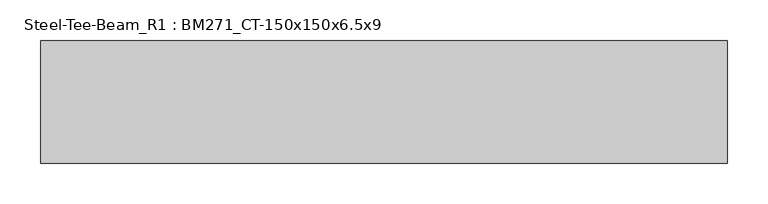
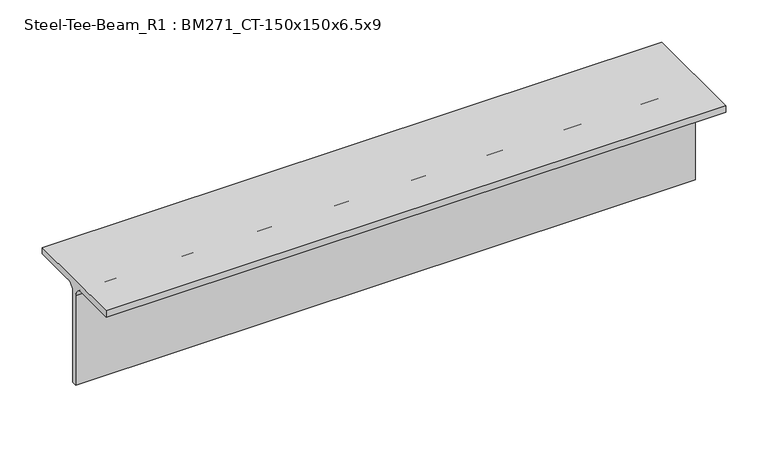
"""IFC4 building model written with IfcOpenShell, lengths in millimetres: member geometry, Steel-Tee-Beam_R1 : BM271_CT-150x150x6.5x9."""

from ifc_helpers import new_model, si_unit, point, frame, frame_2d, origin, place, context, project, spatial, polyline, circle_curve, trimmed, segment, composite_curve, outline, extrude, source, transform, mapped, element, save


def steel_tee_beam_r1_bm271_ct_150x150x6_5x9_ef0092a5(model_context):
    return source(origin(), model_context, "Body", "SweptSolid", [
        extrude(outline(composite_curve([segment(polyline([(75.0, 75.0), (75.0, 66.0), (16.25, 66.0)]), True, "CONTINUOUS"), segment(trimmed(circle_curve(frame_2d((16.25, 53.0)), 13.0), [point((16.25, 66.0))], [point((3.25, 53.0))], True, "CARTESIAN"), True, "CONTINUOUS"), segment(polyline([(3.25, 53.0), (3.25, -75.0), (-3.25, -75.0), (-3.25, 53.0)]), True, "CONTINUOUS"), segment(trimmed(circle_curve(frame_2d((-16.25, 53.0)), 13.0), [point((-3.25, 53.0))], [point((-16.25, 66.0))], True, "CARTESIAN"), True, "CONTINUOUS"), segment(polyline([(-16.25, 66.0), (-75.0, 66.0), (-75.0, 75.0), (75.0, 75.0)]), True, "CONTINUOUS")], self_intersect=False)), frame((-500.0, 0.0, 0.0), z_axis=(1.0, 0.0, 0.0), x_axis=(0.0, 1.0, 0.0)), (0.0, 0.0, 1.0), 841.5608007),
    ])


if __name__ == "__main__":
    model = new_model("IFC4")
    model_context = context("Model", 3, world=origin())
    ifc_project = project(units=[si_unit("LENGTHUNIT", "METRE", prefix="MILLI")], contexts=[model_context])
    site = spatial("IfcSite", under=ifc_project)
    building = spatial("IfcBuilding", under=site)
    placement = place(None, origin())
    steel_tee_beam_r1_bm271_ct_150x150x6_5x9_shape = steel_tee_beam_r1_bm271_ct_150x150x6_5x9_ef0092a5(model_context)
    element("IfcMember", 1, ObjectType="Steel-Tee-Beam_R1 : BM271_CT-150x150x6.5x9", at=placement, inside=building, context=model_context, shape_type="MappedRepresentation", body=[
        mapped(steel_tee_beam_r1_bm271_ct_150x150x6_5x9_shape, transform((0.0, 0.0, 0.0), x_axis=(1.0, 0.0, 0.0), y_axis=(0.0, 1.0, 0.0), z_axis=(0.0, 0.0, 1.0))),
    ])
    save(model, "model.ifc")

# Revit data of these elements
# Type "Steel-Tee-Beam_R1 : BM271_CT-150x150x6.5x9"
#   Keynote = "CT-150x150x6.5x9"
#   Surface Area = 0.588841 m²/m
#   Section Area = 23.3904 cm²
#   Mass per Unit Length = 18.3614 kg/m
#   Length [instance default] = 1.5240 m
#   bf = 0.1500 m
#   d = 0.1500 m
#   k = 0.0220 m
#   r = 0.0130 m
#   tf = 0.0090 m
#   tw = 0.0065 m
#   hec_material4 [instance default] = none
#   hec_material3 [instance default] = none
#   hec_material2 [instance default] = none
#   hec_material1 [instance default] = none
#   Structural Material [instance default] = Steel, 45-345
#   Assembly Code = ""
# Element 1 (IfcMember, "Steel-Tee-Beam_R1 : BM271_CT-150x150x6.5x9")
#   Structural Material = none
# Materials
#   "Steel, 45-345": class "Metal", colour RGB 189 187 185, transparency 0, Description = "Steel 345 MPa", Cost = 0
